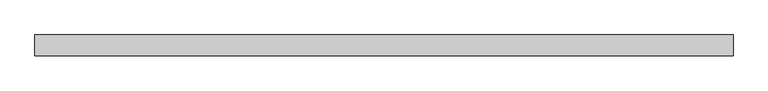
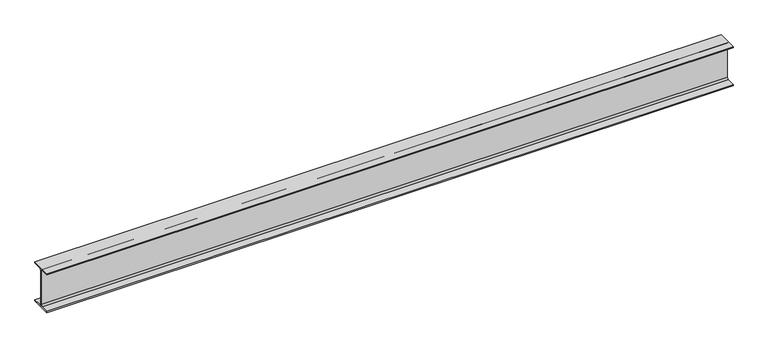
"""IFC4 building model written with IfcOpenShell, lengths in millimetres: beam geometry, 0912_Steel Framing_H-KSD3502 : H_SB_ASB_H-350x175x7x11."""

from ifc_helpers import new_model, si_unit, point, frame, frame_2d, origin, place, context, project, spatial, polyline, circle_curve, trimmed, segment, composite_curve, outline, extrude, source, transform, mapped, element, save


def beam_7925b25c(model_context):
    return source(origin(), model_context, "Body", "SweptSolid", [
        extrude(outline(composite_curve([segment(polyline([(87.5, -164.0), (87.5, -175.0), (-87.5, -175.0), (-87.5, -164.0), (-17.5, -164.0)]), True, "CONTINUOUS"), segment(trimmed(circle_curve(frame_2d((-17.5, -150.0)), 14.0), [point((-17.5, -164.0))], [point((-3.5, -150.0))], True, "CARTESIAN"), True, "CONTINUOUS"), segment(polyline([(-3.5, -150.0), (-3.5, 150.0)]), True, "CONTINUOUS"), segment(trimmed(circle_curve(frame_2d((-17.5, 150.0)), 14.0), [point((-3.5, 150.0))], [point((-17.5, 164.0))], True, "CARTESIAN"), True, "CONTINUOUS"), segment(polyline([(-17.5, 164.0), (-87.5, 164.0), (-87.5, 175.0), (87.5, 175.0), (87.5, 164.0), (17.5, 164.0)]), True, "CONTINUOUS"), segment(trimmed(circle_curve(frame_2d((17.5, 150.0)), 14.0), [point((17.5, 164.0))], [point((3.5, 150.0))], True, "CARTESIAN"), True, "CONTINUOUS"), segment(polyline([(3.5, 150.0), (3.5, -150.0)]), True, "CONTINUOUS"), segment(trimmed(circle_curve(frame_2d((17.5, -150.0)), 14.0), [point((3.5, -150.0))], [point((17.5, -164.0))], True, "CARTESIAN"), True, "CONTINUOUS"), segment(polyline([(17.5, -164.0), (87.5, -164.0)]), True, "CONTINUOUS")], self_intersect=False)), frame((-2920.1382551, 0.0, 0.0), z_axis=(1.0, 0.0, 0.0), x_axis=(0.0, 1.0, 0.0)), (0.0, 0.0, 1.0), 5810.1551285),
    ])


if __name__ == "__main__":
    model = new_model("IFC4")
    model_context = context("Model", 3, world=origin())
    ifc_project = project(units=[si_unit("LENGTHUNIT", "METRE", prefix="MILLI")], contexts=[model_context])
    site = spatial("IfcSite", under=ifc_project)
    building = spatial("IfcBuilding", under=site)
    placement = place(None, origin())
    beam_shape = beam_7925b25c(model_context)
    element("IfcBeam", 1, ObjectType="0912_Steel Framing_H-KSD3502 : H_SB_ASB_H-350x175x7x11", at=placement, inside=building, context=model_context, shape_type="MappedRepresentation", body=[
        mapped(beam_shape, transform((0.0, 0.0, 0.0), x_axis=(1.0, 0.0, 0.0), y_axis=(0.0, 1.0, 0.0), z_axis=(0.0, 0.0, 1.0))),
    ])
    save(model, "model.ifc")

# Revit data of these elements
# Type "0912_Steel Framing_H-KSD3502 : H_SB_ASB_H-350x175x7x11"
#   H_WM Code_1 = "S01AA002-00001 | Main Steel Structure Fabrication Work | Shelter/Building | Medium Steel - Standard (90KG/M>Weight≥30KG/M) | Material: (   )"
#   H_WM Code_2 = "S03AA028-00001 | Main Steel Structure Erection Work | Shelter/Building | Medium Steel (90KG/M>Weight≥30KG/M) | Material: (   )"
#   H_WM Code_3 = "S01AA010-00001 | Main Steel Structure Fabrication Work | Shelter/Building | Steel Painting/Coating | for Non-Fireproofed Steel Surface, Surface Preparation, Primer, Second & Final Coat | Material: (   )"
#   H_Q'ty Cal Type Tag = "SB-Q2"
#   Width = 17.5 cm
#   Web Thickness = 0.7 cm
#   Web Fillet = 1.4 cm
#   Warping Constant = 282000.0 cm⁶
#   W = 0
#   Torsional Moment of Inertia = 19.4042 cm⁴
#   Section Area = 63.14 cm²
#   Plastic Modulus weak axis = 174.0 cm³
#   Plastic Modulus strong axis = 868.0 cm³
#   Perimeter = 1.36 m²/m
#   Nominal Weight = 49.60 kgf/m
#   Moment of Inertia weak axis = 984.00 cm⁴
#   Moment of Inertia strong axis = 13600.00 cm⁴
#   Height = 35.0 cm
#   Flange Thickness = 1.1 cm
#   Elastic Modulus weak axis = 112.0 cm³
#   Elastic Modulus strong axis = 775.0 cm³
#   Centroid Vertical = 17.5 cm
#   Centroid Horizontal = 8.75 cm
#   Ix = 136000000
#   Length [instance default] = 1.5240 m
#   Zx = 868000
#   b = 0.1750 m
#   h = 0.3500 m
#   r = 0.0140 m
#   s = 0.0070 m
#   t = 0.0110 m
#   A = 0.006314 m²
#   Structural Material [instance default] = Steel, 45-345
#   Assembly Code = ""
# Element 1 (IfcBeam, "0912_Steel Framing_H-KSD3502 : H_SB_ASB_H-350x175x7x11")
#   Structural Material = none
# Materials
#   "Steel, 45-345": class "Metal", colour RGB 189 187 185, transparency 0, Description = "Steel 345 MPa", Cost = 0
